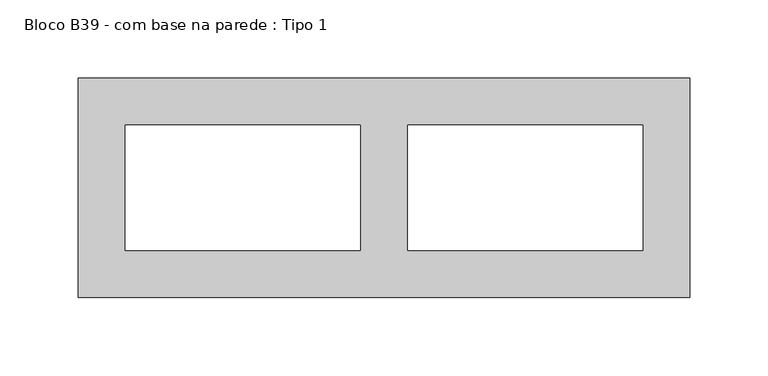
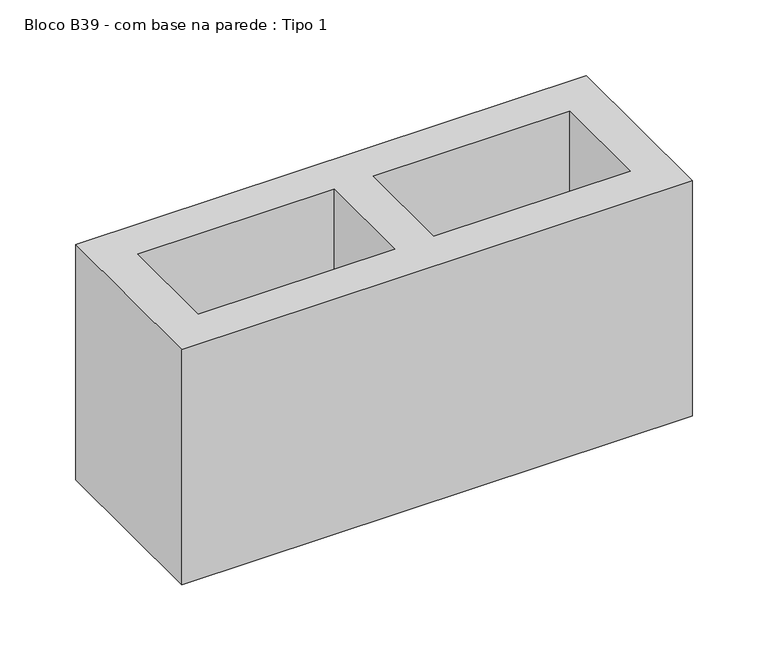
"""IFC4 building model written with IfcOpenShell, lengths in millimetres: proxy geometry, Bloco B39 - com base na parede : Tipo 1."""

from ifc_helpers import new_model, si_unit, origin, origin_with_axes, place, context, project, spatial, polyline, outline, extrude, source, transform, mapped, element, save


def bloco_b39_com_base_na_parede_tipo_1_a9c46908(model_context):
    return source(origin(), model_context, "Body", "SweptSolid", [
        extrude(outline(polyline([(320.0, -70.0), (-70.0, -70.0), (-70.0, 70.0), (320.0, 70.0), (320.0, -70.0)]), holes=[polyline([(110.0, -40.0), (110.0, 40.0), (-40.0, 40.0), (-40.0, -40.0), (110.0, -40.0)]), polyline([(140.0, -40.0), (290.0, -40.0), (290.0, 40.0), (140.0, 40.0), (140.0, -40.0)])]), origin_with_axes(), (0.0, 0.0, 1.0), 190.0),
    ])


if __name__ == "__main__":
    model = new_model("IFC4")
    model_context = context("Model", 3, world=origin())
    ifc_project = project(units=[si_unit("LENGTHUNIT", "METRE", prefix="MILLI")], contexts=[model_context])
    site = spatial("IfcSite", under=ifc_project)
    building = spatial("IfcBuilding", under=site)
    placement = place(None, origin())
    bloco_b39_com_base_na_parede_tipo_1_shape = bloco_b39_com_base_na_parede_tipo_1_a9c46908(model_context)
    element("IfcBuildingElementProxy", 1, Name="Bloco B39 - com base na parede : Tipo 1", ObjectType="Bloco B39 - com base na parede : Tipo 1", at=placement, inside=building, context=model_context, shape_type="MappedRepresentation", body=[
        mapped(bloco_b39_com_base_na_parede_tipo_1_shape, transform((0.0, 0.0, 0.0), x_axis=(1.0, 0.0, 0.0), y_axis=(0.0, 1.0, 0.0), z_axis=(0.0, 0.0, 1.0))),
    ])
    save(model, "model.ifc")

# Revit data of these elements
# Type "Bloco B39 - com base na parede : Tipo 1"
#   SINAPI = ""
#   Assembly Code = ""
